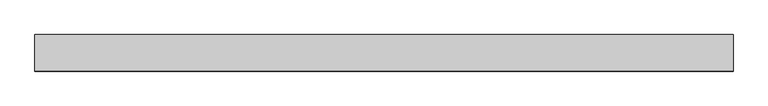
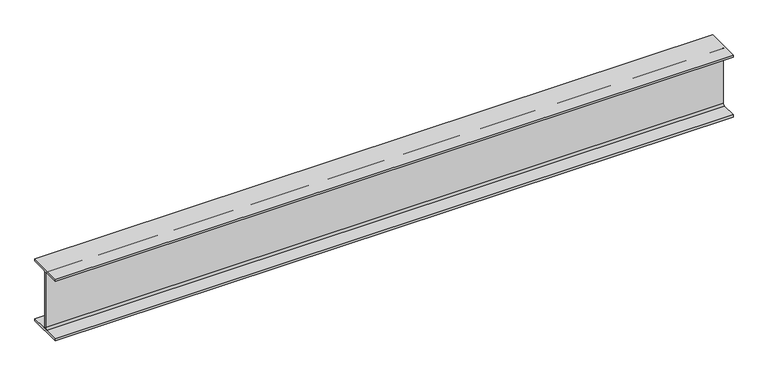
"""IFC4 building model written with IfcOpenShell, lengths in millimetres: beam geometry, Old_Steel Beam_H-KSD3502 : H_SB_ASB_H-250×125x6x9."""

from ifc_helpers import new_model, si_unit, point, frame, frame_2d, origin, place, context, project, spatial, polyline, circle_curve, trimmed, segment, composite_curve, outline, extrude, source, transform, mapped, element, save


def beam_b50dc640(model_context):
    return source(origin(), model_context, "Body", "SweptSolid", [
        extrude(outline(composite_curve([segment(polyline([(82.5, -141.5), (82.5, -151.7), (-82.5, -151.7), (-82.5, -141.5), (-11.9, -141.5)]), True, "CONTINUOUS"), segment(trimmed(circle_curve(frame_2d((-11.9, -132.6)), 8.9), [point((-11.9, -141.5))], [point((-3.0, -132.6))], True, "CARTESIAN"), True, "CONTINUOUS"), segment(polyline([(-3.0, -132.6), (-3.0, 132.6)]), True, "CONTINUOUS"), segment(trimmed(circle_curve(frame_2d((-11.9, 132.6)), 8.9), [point((-3.0, 132.6))], [point((-11.9, 141.5))], True, "CARTESIAN"), True, "CONTINUOUS"), segment(polyline([(-11.9, 141.5), (-82.5, 141.5), (-82.5, 151.7), (82.5, 151.7), (82.5, 141.5), (11.9, 141.5)]), True, "CONTINUOUS"), segment(trimmed(circle_curve(frame_2d((11.9, 132.6)), 8.9), [point((11.9, 141.5))], [point((3.0, 132.6))], True, "CARTESIAN"), True, "CONTINUOUS"), segment(polyline([(3.0, 132.6), (3.0, -132.6)]), True, "CONTINUOUS"), segment(trimmed(circle_curve(frame_2d((11.9, -132.6)), 8.9), [point((3.0, -132.6))], [point((11.9, -141.5))], True, "CARTESIAN"), True, "CONTINUOUS"), segment(polyline([(11.9, -141.5), (82.5, -141.5)]), True, "CONTINUOUS")], self_intersect=False)), frame((-1494.4958478, 0.0, 0.0), z_axis=(1.0, 0.0, 0.0), x_axis=(0.0, 1.0, 0.0)), (0.0, 0.0, 1.0), 3149.2958913),
    ])


if __name__ == "__main__":
    model = new_model("IFC4")
    model_context = context("Model", 3, world=origin())
    ifc_project = project(units=[si_unit("LENGTHUNIT", "METRE", prefix="MILLI")], contexts=[model_context])
    site = spatial("IfcSite", under=ifc_project)
    building = spatial("IfcBuilding", under=site)
    placement = place(None, origin())
    beam_shape = beam_b50dc640(model_context)
    element("IfcBeam", 1, ObjectType="Old_Steel Beam_H-KSD3502 : H_SB_ASB_H-250×125x6x9", at=placement, inside=building, context=model_context, shape_type="MappedRepresentation", body=[
        mapped(beam_shape, transform((0.0, 0.0, 0.0), x_axis=(1.0, 0.0, 0.0), y_axis=(0.0, 1.0, 0.0), z_axis=(0.0, 0.0, 1.0))),
    ])
    save(model, "model.ifc")

# Revit data of these elements
# Type "Old_Steel Beam_H-KSD3502 : H_SB_ASB_H-250×125x6x9"
#   Width = 12.5 cm
#   Web Thickness = 0.6 cm
#   Web Fillet = 1.2 cm
#   Warping Constant = 42539.8 cm⁶
#   Torsional Moment of Inertia = 7.8102 cm⁴
#   Torsional Modulus = 1.0 cm³
#   Section Area = 37.66 cm²
#   Plastic Modulus weak axis = 73.1 cm³
#   Plastic Modulus strong axis = 366.0 cm³
#   Perimeter = 0.97 m²/m
#   Nominal Weight = 29.60 kgf/m
#   Moment of Inertia weak axis = 294.00 cm⁴
#   Moment of Inertia strong axis = 4050.00 cm⁴
#   Height = 25.0 cm
#   Flange Thickness = 0.9 cm
#   Elastic Modulus weak axis = 47.0 cm³
#   Elastic Modulus strong axis = 324.0 cm³
#   Centroid Vertical = 12.5 cm
#   Centroid Horizontal = 6.25 cm
#   Length [instance default] = 1.5240 m
#   Structural Material [instance default] = Steel, 45-345
#   Assembly Code = ""
# Element 1 (IfcBeam, "Old_Steel Beam_H-KSD3502 : H_SB_ASB_H-250×125x6x9")
#   Structural Material = none
# Materials
#   "Steel, 45-345": class "Metal", colour RGB 189 187 185, transparency 0, Description = "Steel 345 MPa", Cost = 0
